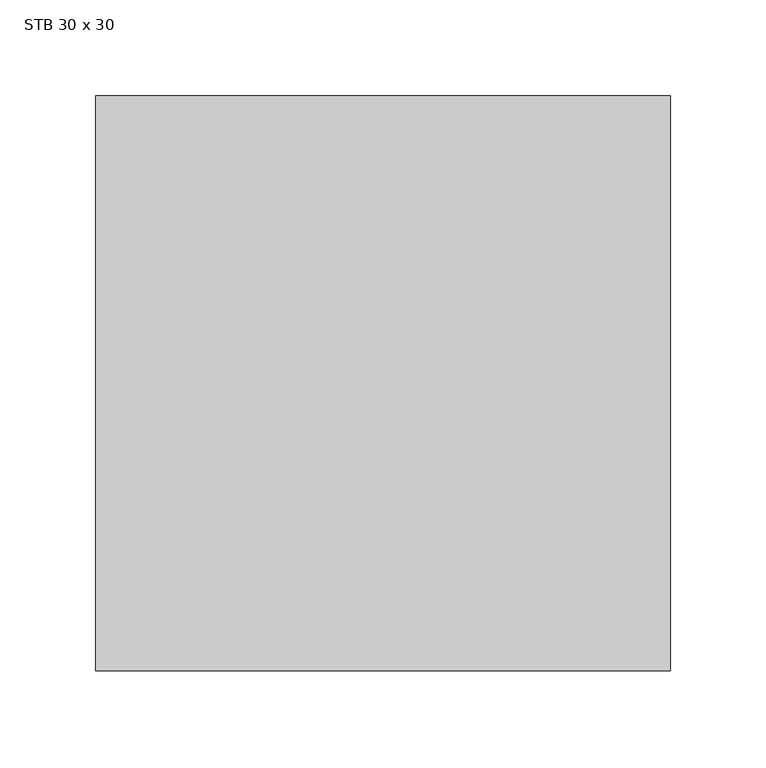
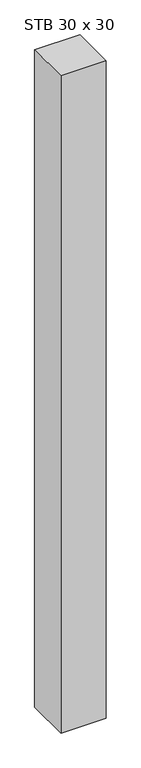
"""IFC4 building model written with IfcOpenShell, lengths in millimetres: column geometry, STB Stütze - rechteckig : STB 30 x 30."""

from ifc_helpers import new_model, si_unit, frame, origin, place, context, project, spatial, polyline, outline, extrude, source, transform, mapped, element, save


def stb_30_x_30_c50efebe(model_context):
    return source(origin(), model_context, "Body", "SweptSolid", [
        extrude(outline(polyline([(150.0, 150.0), (150.0, -150.0), (-150.0, -150.0), (-150.0, 150.0), (150.0, 150.0)])), frame((0.0, 0.0, -1570.0), z_axis=(0.0, 0.0, 1.0), x_axis=(1.0, 0.0, 0.0)), (0.0, 0.0, 1.0), 4600.0),
    ])


if __name__ == "__main__":
    model = new_model("IFC4")
    model_context = context("Model", 3, world=origin())
    ifc_project = project(units=[si_unit("LENGTHUNIT", "METRE", prefix="MILLI")], contexts=[model_context])
    site = spatial("IfcSite", under=ifc_project)
    building = spatial("IfcBuilding", under=site)
    placement = place(None, origin())
    stb_30_x_30_shape = stb_30_x_30_c50efebe(model_context)
    element("IfcColumn", 1, ObjectType="STB Stütze - rechteckig : STB 30 x 30", at=placement, inside=building, context=model_context, shape_type="MappedRepresentation", body=[
        mapped(stb_30_x_30_shape, transform((0.0, 0.0, 0.0), x_axis=(1.0, 0.0, 0.0), y_axis=(0.0, 1.0, 0.0), z_axis=(0.0, 0.0, 1.0))),
    ])
    save(model, "model.ifc")

# Revit data of these elements
# Type "STB Stütze - rechteckig : STB 30 x 30"
#   Breite = 0.300 m
#   Tiefe = 0.300 m
#   Structural Material [instance default] = Stahlbeton - Ortbeton
# Element 1 (IfcColumn, "STB Stütze - rechteckig : STB 30 x 30")
#   Materials on its faces: "Stahlbeton - Ortbeton"
# Materials
#   "Stahlbeton - Ortbeton": class "Beton", colour RGB 247 247 247, transparency 0, Cost = 0
